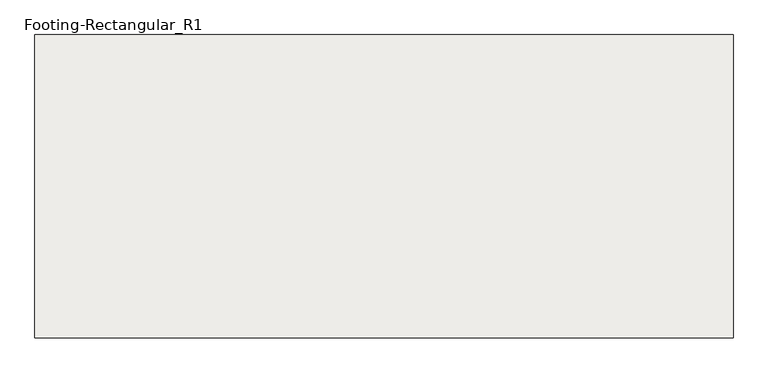
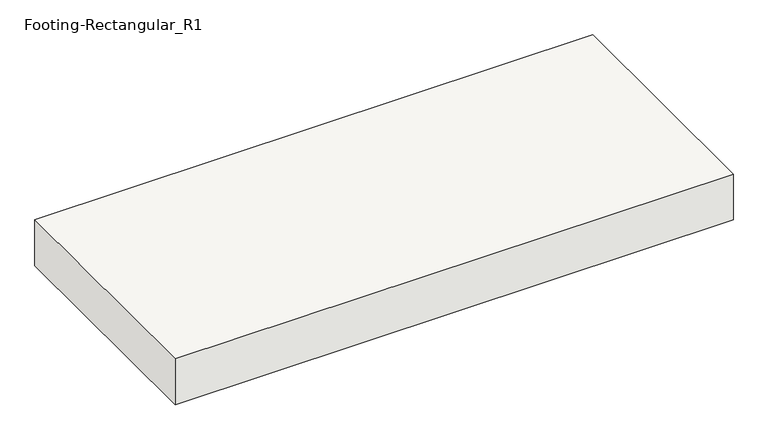
"""IFC4 building model written with IfcOpenShell, lengths in millimetres: slab geometry, Footing-Rectangular_R1 : H_SF_AR_S18_W5750xL2500xT500_Bitumen_F6."""

import ifcopenshell
import ifcopenshell.guid

model = None  # the IFC model being written
_history = None  # IfcOwnerHistory: only IFC2X3 demands one
_inside = {}  # id of a spatial element -> (the spatial element, [elements in it])
_under = {}  # id of a project, library or spatial element -> (it, [spatial elements below it])
_declared = {}  # id of a project -> (the project, [libraries it declares])
_typed = {}  # id of a type object -> (the type object, [elements of that type])
_made_of = {}  # id of a material, layer set ... -> (it, [elements and type objects made of it])


def new_model(schema):
    """Start an empty IFC model of exactly this schema.

    Asked for "IFC4X3", IfcOpenShell would pick the latest addendum, in which some entities
    have other attributes; the version numbers below select the first issue.
    IFC2X3 requires an IfcOwnerHistory on every rooted entity: one is made here for all.
    """
    global model, _history
    if schema == "IFC4X3":
        model = ifcopenshell.file(schema_version=(4, 3, 0, 0))
    else:
        model = ifcopenshell.file(schema=schema)
    _inside.clear()
    _under.clear()
    _declared.clear()
    _typed.clear()
    _made_of.clear()
    _history = None
    if model.schema == "IFC2X3":
        org = make("IfcOrganization", Name="unknown")
        user = make(
            "IfcPersonAndOrganization",
            ThePerson=make("IfcPerson", FamilyName="unknown"),
            TheOrganization=org,
        )
        app = make(
            "IfcApplication",
            ApplicationDeveloper=org,
            Version="unknown",
            ApplicationFullName="unknown",
            ApplicationIdentifier="unknown",
        )
        _history = make(
            "IfcOwnerHistory",
            OwningUser=user,
            OwningApplication=app,
            ChangeAction="ADDED",
            CreationDate=0,
        )
    return model


def make(cls, **values):
    """One entity of the class cls with the attributes given. An attribute that is None is left unset."""
    return model.create_entity(
        cls, **{name: value for name, value in values.items() if value is not None}
    )


def rooted(cls, **values):
    """An entity with a GlobalId (a new one), such as an element, a storey or a relation."""
    return make(cls, GlobalId=ifcopenshell.guid.new(), OwnerHistory=_history, **values)


def si_unit(unit_type, name, prefix=None):
    """IfcSIUnit, for example si_unit("LENGTHUNIT", "METRE", prefix="MILLI")."""
    return make("IfcSIUnit", UnitType=unit_type, Prefix=prefix, Name=name)


def assignment(units):
    """IfcUnitAssignment: the units of a project."""
    return None if units is None else make("IfcUnitAssignment", Units=units)


def point(xyz):
    """IfcCartesianPoint."""
    return None if xyz is None else make("IfcCartesianPoint", Coordinates=xyz)


def direction(xyz):
    """IfcDirection."""
    return None if xyz is None else make("IfcDirection", DirectionRatios=xyz)


def frame(location, z_axis=None, x_axis=None):
    """IfcAxis2Placement3D, a coordinate frame: its origin and axes. An axis left out is left unset."""
    return make(
        "IfcAxis2Placement3D",
        Location=point(location),
        Axis=direction(z_axis),
        RefDirection=direction(x_axis),
    )


def origin():
    """The frame at (0, 0, 0) with its axes left unset."""
    return frame((0.0, 0.0, 0.0))


def place(relative_to, where):
    """IfcLocalPlacement: puts the frame where relative to a parent placement (None: the world)."""
    return make(
        "IfcLocalPlacement", PlacementRelTo=relative_to, RelativePlacement=where
    )


def context(
    kind, dimensions, precision=None, world=None, true_north=None, identifier=None
):
    """IfcGeometricRepresentationContext, for example the 3D "Model" context."""
    return make(
        "IfcGeometricRepresentationContext",
        ContextIdentifier=identifier,
        ContextType=kind,
        CoordinateSpaceDimension=dimensions,
        Precision=precision,
        WorldCoordinateSystem=world,
        TrueNorth=true_north,
    )


def project(units=None, contexts=None):
    """IfcProject with its units and contexts."""
    return rooted(
        "IfcProject",
        Name="project",
        RepresentationContexts=contexts,
        UnitsInContext=assignment(units),
    )


def spatial(cls, under=None, at=None, **own):
    """A site, building, storey or space (cls), placed at a placement, below another one or the project."""
    s = rooted(cls, ObjectPlacement=at, **own)
    if under is not None:
        _under.setdefault(under.id(), (under, []))[1].append(s)
    return s


def polyline(points):
    """IfcPolyline through the points."""
    return make("IfcPolyline", Points=[point(p) for p in points])


def outline(outer, holes=None, kind="AREA"):
    """IfcArbitraryClosedProfileDef: a profile drawn as a closed curve; with holes, ...WithVoids."""
    if holes is None:
        return make("IfcArbitraryClosedProfileDef", ProfileType=kind, OuterCurve=outer)
    return make(
        "IfcArbitraryProfileDefWithVoids",
        ProfileType=kind,
        OuterCurve=outer,
        InnerCurves=holes,
    )


def extrude(swept, where, along, depth):
    """IfcExtrudedAreaSolid: the profile swept, set in the frame where, extruded along a direction by depth."""
    return make(
        "IfcExtrudedAreaSolid",
        SweptArea=swept,
        Position=where,
        ExtrudedDirection=direction(along),
        Depth=depth,
    )


def shape(context_of_items, identifier, shape_type, items):
    """IfcShapeRepresentation: the items that make up one representation, for example the "Body"."""
    return make(
        "IfcShapeRepresentation",
        ContextOfItems=context_of_items,
        RepresentationIdentifier=identifier,
        RepresentationType=shape_type,
        Items=items,
    )


def source(mapping_origin, context_of_items, identifier, shape_type, items):
    """IfcRepresentationMap: a shape defined once, which mapped items show again and again."""
    return make(
        "IfcRepresentationMap",
        MappingOrigin=mapping_origin,
        MappedRepresentation=shape(context_of_items, identifier, shape_type, items),
    )


def transform(
    local_origin,
    x_axis=None,
    y_axis=None,
    z_axis=None,
    scale=None,
    scale2=None,
    scale3=None,
    uniform=True,
):
    """IfcCartesianTransformationOperator3D, or its non-uniform kind. x_axis, y_axis, z_axis: its Axis1, 2, 3."""
    if uniform:
        return make(
            "IfcCartesianTransformationOperator3D",
            Axis1=direction(x_axis),
            Axis2=direction(y_axis),
            LocalOrigin=point(local_origin),
            Scale=scale,
            Axis3=direction(z_axis),
        )
    return make(
        "IfcCartesianTransformationOperator3DnonUniform",
        Axis1=direction(x_axis),
        Axis2=direction(y_axis),
        LocalOrigin=point(local_origin),
        Scale=scale,
        Axis3=direction(z_axis),
        Scale2=scale2,
        Scale3=scale3,
    )


def mapped(mapping_source, mapping_target):
    """IfcMappedItem: shows the shape of a source again, moved by a transform."""
    return make(
        "IfcMappedItem", MappingSource=mapping_source, MappingTarget=mapping_target
    )


def made_of(thing, what):
    """Note that an element or type object is made of a material, layer set ...; save() writes the relation."""
    if what is not None:
        _made_of.setdefault(what.id(), (what, []))[1].append(thing)
    return thing


def element(
    cls,
    number,
    at=None,
    inside=None,
    cuts=None,
    type_object=None,
    material=None,
    context=None,
    identifier="Body",
    shape_type=None,
    held_by="IfcProductDefinitionShape",
    body=None,
    shapes=None,
    **own,
):
    """One element of the class cls, such as IfcWall. Its Tag is "e" and its number.

    at: its placement. inside: the storey or other place that contains it. cuts: it is an
    opening in that element (IfcRelVoidsElement). A single representation is given by context,
    identifier, shape_type and body (its items); several are given by shapes. held_by: the class
    of the entity that holds the representations. save() writes the other relations.
    """
    e = rooted(cls, Tag="e%d" % number, ObjectPlacement=at, **own)
    if body is not None:
        shapes = [shape(context, identifier, shape_type, body)]
    if shapes is not None:
        e.Representation = make(held_by, Representations=shapes)
    if inside is not None:
        _inside.setdefault(inside.id(), (inside, []))[1].append(e)
    if cuts is not None:
        rooted(
            "IfcRelVoidsElement", RelatingBuildingElement=cuts, RelatedOpeningElement=e
        )
    if type_object is not None:
        _typed.setdefault(type_object.id(), (type_object, []))[1].append(e)
    return made_of(e, material)


def aggregate(whole, parts):
    """IfcRelAggregates: a whole, such as a stair, and the parts it consists of."""
    return rooted("IfcRelAggregates", RelatingObject=whole, RelatedObjects=parts)


def save(model, path):
    """Write the relations noted so far, then the file.

    IfcRelAggregates (storeys below a building ...), IfcRelContainedInSpatialStructure (elements
    in a storey), IfcRelDefinesByType, IfcRelAssociatesMaterial and IfcRelDeclares: one each for
    every whole, place, type object, material and project.
    """
    for whole, parts in _under.values():
        aggregate(whole, parts)
    for where, things in _inside.values():
        rooted(
            "IfcRelContainedInSpatialStructure",
            RelatedElements=things,
            RelatingStructure=where,
        )
    for kind, things in _typed.values():
        rooted("IfcRelDefinesByType", RelatedObjects=things, RelatingType=kind)
    for what, things in _made_of.values():
        rooted("IfcRelAssociatesMaterial", RelatedObjects=things, RelatingMaterial=what)
    for by, libraries in _declared.values():
        rooted("IfcRelDeclares", RelatingContext=by, RelatedDefinitions=libraries)
    model.write(path)


def footing_rectangular_r1_f7e30f5b(model_context):
    return source(origin(), model_context, "Body", "SweptSolid", [
        extrude(outline(polyline([(2875.0, 1250.0), (2875.0, -1250.0), (-2875.0, -1250.0), (-2875.0, 1250.0), (2875.0, 1250.0)])), frame((0.0, 0.0, -500.0), z_axis=(0.0, 0.0, 1.0), x_axis=(1.0, 0.0, 0.0)), (0.0, 0.0, 1.0), 500.0),
    ])


if __name__ == "__main__":
    model = new_model("IFC4")
    model_context = context("Model", 3, world=origin())
    ifc_project = project(units=[si_unit("LENGTHUNIT", "METRE", prefix="MILLI")], contexts=[model_context])
    site = spatial("IfcSite", under=ifc_project)
    building = spatial("IfcBuilding", under=site)
    placement = place(None, origin())
    footing_rectangular_r1_shape = footing_rectangular_r1_f7e30f5b(model_context)
    element("IfcSlab", 1, ObjectType="Footing-Rectangular_R1 : H_SF_AR_S18_W5750xL2500xT500_Bitumen_F6", at=placement, inside=building, context=model_context, shape_type="MappedRepresentation", body=[
        mapped(footing_rectangular_r1_shape, transform((0.0, 0.0, 0.0), x_axis=(1.0, 0.0, 0.0), y_axis=(0.0, 1.0, 0.0), z_axis=(0.0, 0.0, 1.0))),
    ])
    save(model, "model.ifc")

# Revit data of these elements
# Type "Footing-Rectangular_R1 : H_SF_AR_S18_W5750xL2500xT500_Bitumen_F6"
#   Type Mark = "F6"
#   Top bar = "D25@300"
#   Description = "UG Shallow Foundation"
#   Bottom bar = "D20@300"
#   Width = 5750 mm
#   Length = 2500 mm
#   Foundation Thickness = 500 mm
#   Structural Material [instance default] = none
#   Assembly Code = ""
